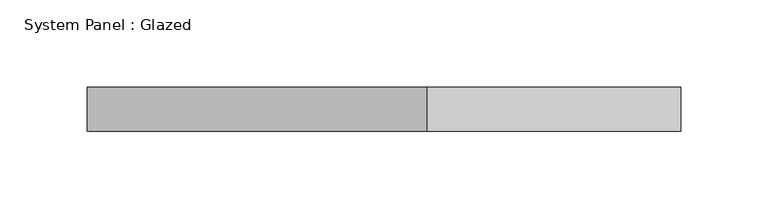
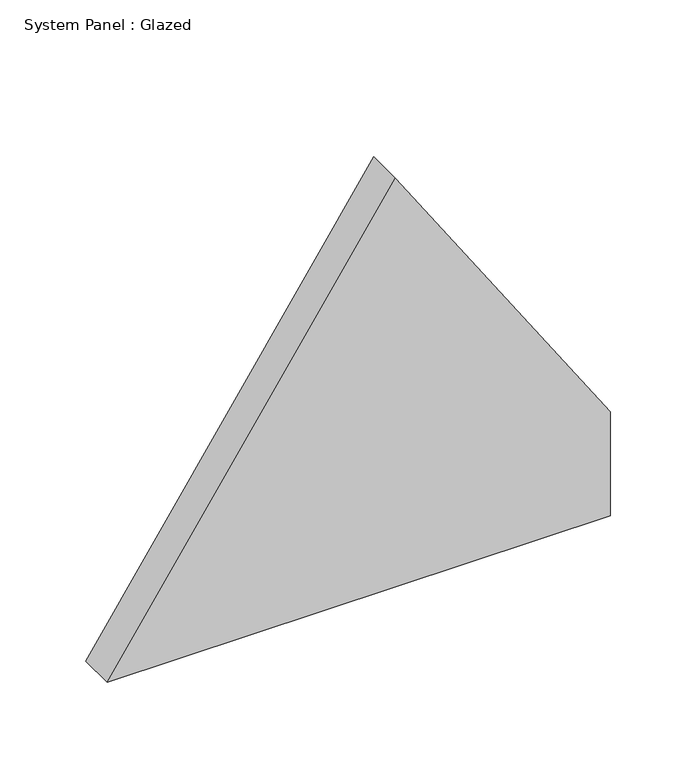
"""IFC4 building model written with IfcOpenShell, lengths in millimetres: plate geometry, System Panel : Glazed."""

from ifc_helpers import new_model, si_unit, frame, origin, place, context, project, spatial, polyline, outline, extrude, source, transform, mapped, element, save


def system_panel_glazed_70284913(model_context):
    return source(origin(), model_context, "Body", "SweptSolid", [
        extrude(outline(polyline([(0.0, -169.6975445), (0.0, 169.6975445), (74.0824486, 169.6975445), (291.5525508, 24.6975445), (0.0, -169.6975445)])), frame((0.0, 24.5, 0.0), z_axis=(0.0, 1.0, 0.0), x_axis=(0.0, 0.0, 1.0)), (0.0, 0.0, 1.0), 25.0),
    ])


if __name__ == "__main__":
    model = new_model("IFC4")
    model_context = context("Model", 3, world=origin())
    ifc_project = project(units=[si_unit("LENGTHUNIT", "METRE", prefix="MILLI")], contexts=[model_context])
    site = spatial("IfcSite", under=ifc_project)
    building = spatial("IfcBuilding", under=site)
    placement = place(None, origin())
    system_panel_glazed_shape = system_panel_glazed_70284913(model_context)
    element("IfcPlate", 1, ObjectType="System Panel : Glazed", at=placement, inside=building, context=model_context, shape_type="MappedRepresentation", body=[
        mapped(system_panel_glazed_shape, transform((0.0, 0.0, 0.0), x_axis=(1.0, 0.0, 0.0), y_axis=(0.0, 1.0, 0.0), z_axis=(0.0, 0.0, 1.0))),
    ])
    save(model, "model.ifc")

# Revit data of these elements
# Type "System Panel : Glazed"
#   Keynote = "H11"
#   Construction Type Id = "GSP4R"
#   Analytic Construction = "1/8 in Pilkington single glazing"
#   Visual Light Transmittance = 0.9
#   Solar Heat Gain Coefficient = 0.86
#   Heat Transfer Coefficient (U) = 6.7069 W/(m²·K)
#   Define Thermal Properties by = 1
# Element 1 (IfcPlate, "System Panel : Glazed")
#   Materials on its faces: "Glass"
# Materials
#   "Glass": class "Glass", colour RGB 0 128 192, transparency 0.9, Description = "Soda Lime Glass", Cost = 0
